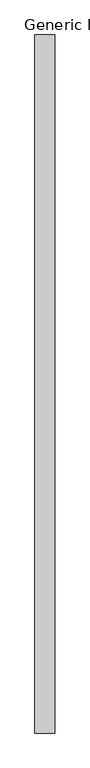
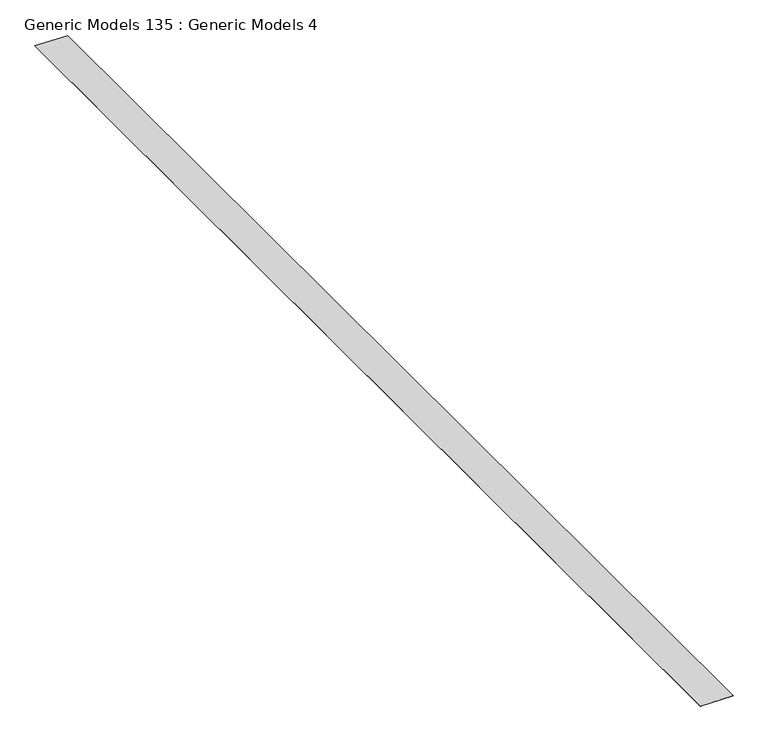
"""IFC4 building model written with IfcOpenShell, lengths in millimetres: proxy geometry, Generic Models 135 : Generic Models 4."""

from ifc_helpers import new_model, si_unit, frame, origin, place, context, project, spatial, polyline, outline, extrude, source, transform, mapped, element, save


def generic_models_135_generic_models_4_0faf0f8a(model_context):
    return source(origin(), model_context, "Body", "SweptSolid", [
        extrude(outline(polyline([(0.0, -533.9447377), (0.0, 0.0), (18643.6, 0.0), (18643.6, -533.9447377), (0.0, -533.9447377)])), frame((7279.5977813, -6864.9230338, 126909.8307553), z_axis=(0.02082881368186553, 0.0, 0.9997830567281115), x_axis=(0.0, 1.0, 0.0)), (0.0, 0.0, 1.0), 0.79375),
    ])


if __name__ == "__main__":
    model = new_model("IFC4")
    model_context = context("Model", 3, world=origin())
    ifc_project = project(units=[si_unit("LENGTHUNIT", "METRE", prefix="MILLI")], contexts=[model_context])
    site = spatial("IfcSite", under=ifc_project)
    building = spatial("IfcBuilding", under=site)
    placement = place(None, origin())
    generic_models_135_generic_models_4_shape = generic_models_135_generic_models_4_0faf0f8a(model_context)
    element("IfcBuildingElementProxy", 1, Name="Generic Models 135 : Generic Models 4", ObjectType="Generic Models 135 : Generic Models 4", at=placement, inside=building, context=model_context, shape_type="MappedRepresentation", body=[
        mapped(generic_models_135_generic_models_4_shape, transform((0.0, 0.0, 0.0), x_axis=(1.0, 0.0, 0.0), y_axis=(0.0, 1.0, 0.0), z_axis=(0.0, 0.0, 1.0))),
    ])
    save(model, "model.ifc")

# Revit data of these elements
# Element 1 (IfcBuildingElementProxy, "Generic Models 135 : Generic Models 4")
#   Materials on its faces: "_HYDROSTOP LIQUID MEMBRANE - FOLLOW MANU. RECOMMENDED INSTALLATION DETAILS"
# Materials
#   "_HYDROSTOP LIQUID MEMBRANE - FOLLOW MANU. RECOMMENDED INSTALLATION DETAILS": class "Generic", colour RGB 156 184 169, transparency 0, Cost = 0
